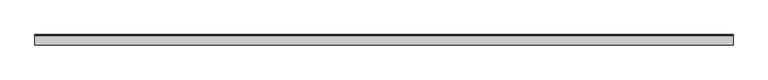
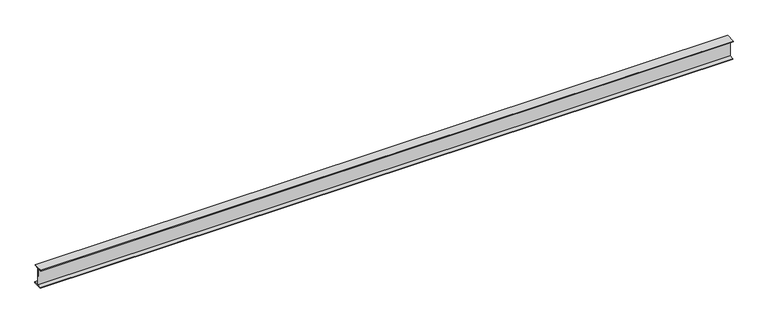
"""IFC4 building model written with IfcOpenShell, lengths in millimetres: proxy geometry, Generic Models 7:Generic Models 1:8:Generic Models 1:8 : Generic Models 7:Generic Models 1:337419:12 : Generic Models 7:Generic Models 1:8:Generic Models 1:8 : Generic Models 7:Generic Models 1:337419:315935."""

from ifc_helpers import new_model, si_unit, frame, origin, place, context, project, spatial, polyline, outline, extrude, source, transform, mapped, element, save


def generic_models_82202dee(model_context):
    return source(origin(), model_context, "Body", "SweptSolid", [
        extrude(outline(polyline([(-575776.1959679, 4050.6710253), (-575776.5189849, 4058.7966924), (-575674.8224487, 4062.8394016), (-575674.5037523, 4054.8224223), (-575722.5330172, 4052.9131306), (-575714.9767791, 3862.8318775), (-575666.9893502, 3864.7395062), (-575666.6738004, 3856.8016819), (-575768.0507072, 3852.7716788), (-575768.3648258, 3860.6735004), (-575720.654098, 3862.5701294), (-575728.2074467, 4052.5786973), (-575776.1959679, 4050.6710253)])), frame((588867.6367239, 0.0, 0.0), z_axis=(1.0, 0.0, 0.0), x_axis=(0.0, 1.0, 0.0)), (0.0, 0.0, 1.0), 7315.2),
    ])


if __name__ == "__main__":
    model = new_model("IFC4")
    model_context = context("Model", 3, world=origin())
    ifc_project = project(units=[si_unit("LENGTHUNIT", "METRE", prefix="MILLI")], contexts=[model_context])
    site = spatial("IfcSite", under=ifc_project)
    building = spatial("IfcBuilding", under=site)
    placement = place(None, origin())
    generic_models_shape = generic_models_82202dee(model_context)
    element("IfcBuildingElementProxy", 1, Name="Generic Models 7:Generic Models 1:8:Generic Models 1:8 : Generic Models 7:Generic Models 1:337419:12 : Generic Models 7:Generic Models 1:8:Generic Models 1:8 : Generic Models 7:Generic Models 1:337419:315935", ObjectType="Generic Models 7:Generic Models 1:8:Generic Models 1:8 : Generic Models 7:Generic Models 1:337419:12 : Generic Models 7:Generic Models 1:8:Generic Models 1:8 : Generic Models 7:Generic Models 1:337419:315935", at=placement, inside=building, context=model_context, shape_type="MappedRepresentation", body=[
        mapped(generic_models_shape, transform((0.0, 0.0, 0.0), x_axis=(1.0, 0.0, 0.0), y_axis=(0.0, 1.0, 0.0), z_axis=(0.0, 0.0, 1.0))),
    ])
    save(model, "model.ifc")

# Revit data of these elements
# Type "Generic Models 7:Generic Models 1:8:Generic Models 1:8 : Generic Models 7:Generic Models 1:337419:12 : Generic Models 7:Generic Models 1:8:Generic Models 1:8 : Generic Models 7:Generic Models 1:337419:315935"
#   NameOverride = "Generic Models 7:Generic Models 1:8:Generic Models 1:8 : Generic Models 7:Generic Models 1:337419:315935"
#   ObjectTypeOverride = "Generic Models 1:8 : Generic Models 7:Generic Models 1:337419"
#   Reference = "Generic Models 1"
#   Tag = "315935"
# Element 1 (IfcBuildingElementProxy, "Generic Models 7:Generic Models 1:8:Generic Models 1:8 : Generic Models 7:Generic Models 1:337419:12 : Generic Models 7:Generic Models 1:8:Generic Models 1:8 : Generic Models 7:Generic Models 1:337419:315935")
#   Materials on its faces: "STRUCTURAL STEEL - SEE STRUCT. DWGS"
# Materials
#   "STRUCTURAL STEEL - SEE STRUCT. DWGS": class "Metal", colour RGB 189 187 185, transparency 0, Description = "Structural steel 50ksi", Cost = 0
